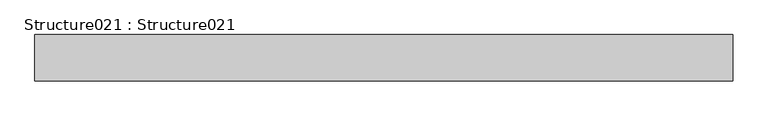
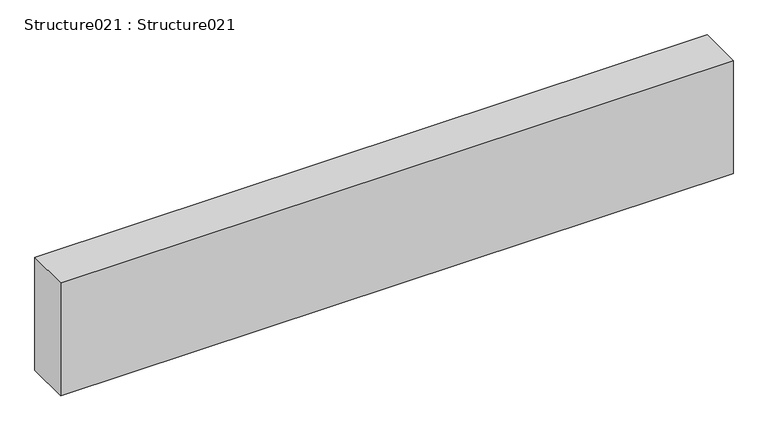
"""IFC4 building model written with IfcOpenShell, lengths in millimetres: proxy geometry, Structure021 : Structure021."""

from ifc_helpers import new_model, si_unit, frame, origin, place, context, project, spatial, polyline, outline, extrude, source, transform, mapped, element, save


def structure021_structure021_672eb29b(model_context):
    return source(origin(), model_context, "Body", "SweptSolid", [
        extrude(outline(polyline([(14383.0178845, -4253.3675368), (14383.0178845, -4386.7175368), (12383.0178845, -4386.7175368), (12383.0178845, -4253.3675368), (14383.0178845, -4253.3675368)])), frame((0.0, 0.0, 39757.096), z_axis=(0.0, 0.0, 1.0), x_axis=(1.0, 0.0, 0.0)), (0.0, 0.0, 1.0), 355.6),
    ])


if __name__ == "__main__":
    model = new_model("IFC4")
    model_context = context("Model", 3, world=origin())
    ifc_project = project(units=[si_unit("LENGTHUNIT", "METRE", prefix="MILLI")], contexts=[model_context])
    site = spatial("IfcSite", under=ifc_project)
    building = spatial("IfcBuilding", under=site)
    placement = place(None, origin())
    structure021_structure021_shape = structure021_structure021_672eb29b(model_context)
    element("IfcBuildingElementProxy", 1, Name="Structure021 : Structure021", ObjectType="Structure021 : Structure021", at=placement, inside=building, context=model_context, shape_type="MappedRepresentation", body=[
        mapped(structure021_structure021_shape, transform((0.0, 0.0, 0.0), x_axis=(1.0, 0.0, 0.0), y_axis=(0.0, 1.0, 0.0), z_axis=(0.0, 0.0, 1.0))),
    ])
    save(model, "model.ifc")

# Revit data of these elements
# Type "Structure021 : Structure021"
#   NameOverride = "Structure021"
# Element 1 (IfcBuildingElementProxy, "Structure021 : Structure021")
#   Materials on its faces: "STRUCTURAL MEMBER (SEE STRUCTURAL DWGS)"
# Materials
#   "STRUCTURAL MEMBER (SEE STRUCTURAL DWGS)": class "Unassigned", colour RGB 176 134 95, transparency 0, Cost = 0
